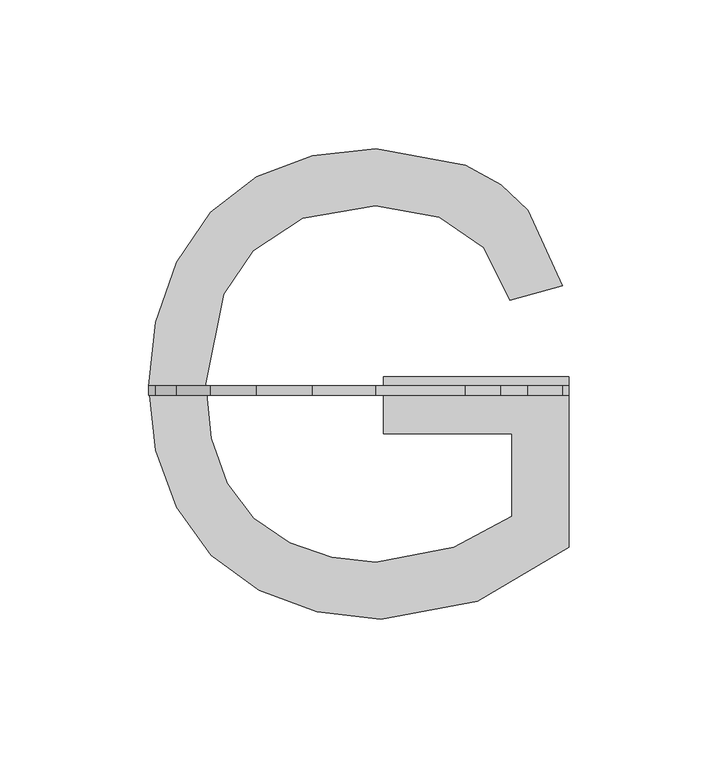
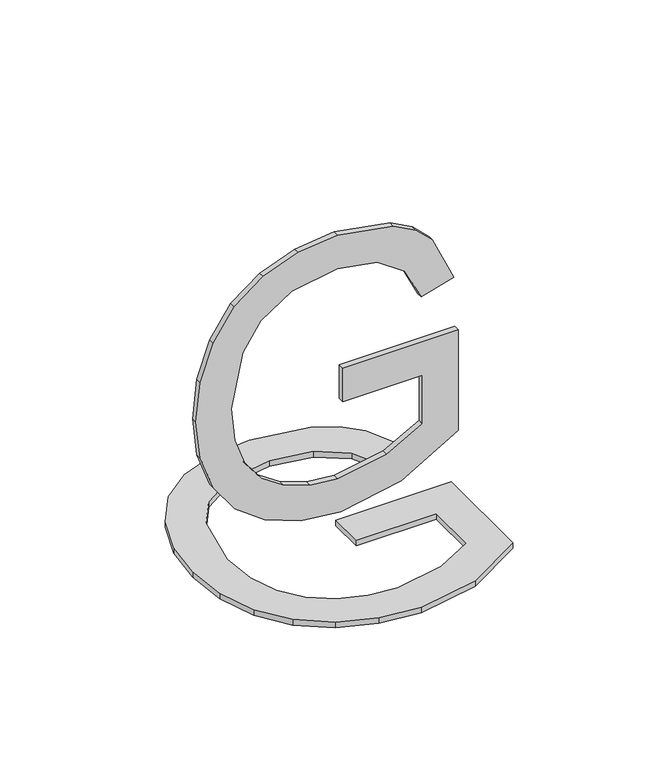
"""IFC4 building model written with IfcOpenShell, lengths in millimetres: proxy geometry, Grid Number1_FedEx : Grid Number1_FedEx."""

from ifc_helpers import new_model, si_unit, frame, origin, origin_with_axes, place, context, project, spatial, polyline, outline, extrude, source, transform, mapped, element, save


def entourage_0d31b632(model_context):
    return source(origin(), model_context, "Body", "SweptSolid", [
        extrude(outline(polyline([(-102.093637, 206.3869621), (-102.093637, 225.5238891), (-39.898624, 225.5238891), (-39.898624, 168.2999919), (-70.603674, 150.2469924), (-103.0654341, 144.191949), (-124.5337398, 146.5980812), (-143.9369766, 153.8164778), (-160.0557262, 165.5948453), (-171.6705702, 181.6808902), (-178.6927385, 200.9766687), (-181.0334612, 222.384237), (-178.7020827, 243.9459847), (-171.707947, 264.0033158), (-160.3407244, 280.8275527), (-144.8900853, 292.690018), (-126.0708611, 299.7262026), (-104.5978833, 302.0715975), (-74.659058, 296.6332715), (-62.721839, 290.1297065), (-53.6719787, 281.4956632), (-42.1038558, 256.1728739), (-59.7457105, 251.2017581), (-68.4731958, 268.899678), (-83.3865433, 279.1035473), (-104.8968978, 282.9346704), (-129.3973972, 278.8045328), (-146.0674548, 267.9652577), (-155.9162444, 253.2201059), (-161.8965342, 223.1691501), (-160.0977751, 204.8685291), (-154.7014981, 189.8103465), (-145.8712266, 178.1020606), (-133.7704841, 169.8511296), (-119.6093449, 164.9594395), (-104.5978833, 163.3288761), (-78.4154274, 168.2439267), (-59.0355511, 178.7281221), (-59.0355511, 206.3869621), (-102.093637, 206.3869621)])), origin_with_axes(), (0.0, 0.0, 1.0), 3.175),
        extrude(outline(polyline([(74.2827904, -102.093637), (74.2827904, -59.0355511), (46.6239505, -59.0355511), (36.1397551, -78.4154274), (31.2247044, -104.5978833), (32.8552678, -119.6093449), (37.7469579, -133.7704841), (45.9978889, -145.8712266), (57.7061748, -154.7014981), (72.7643574, -160.0977751), (91.0649784, -161.8965342), (121.1159342, -155.9162444), (135.861086, -146.0674548), (146.7003611, -129.3973972), (150.8304987, -104.8968978), (146.9993756, -83.3865433), (136.7955063, -68.4731958), (119.0975864, -59.7457105), (124.0687022, -42.1038558), (149.3914915, -53.6719787), (158.0255348, -62.721839), (164.5290998, -74.659058), (169.9674258, -104.5978833), (167.6220309, -126.0708611), (160.5858463, -144.8900853), (148.723381, -160.3407244), (131.8991441, -171.707947), (111.841813, -178.7020827), (90.2800654, -181.0334612), (68.872497, -178.6927385), (49.5767185, -171.6705702), (33.4906736, -160.0557262), (21.7123061, -143.9369766), (14.4939095, -124.5337398), (12.0877774, -103.0654341), (18.1428207, -70.603674), (36.1958203, -39.898624), (93.4197175, -39.898624), (93.4197175, -102.093637), (74.2827904, -102.093637)])), frame((0.0, 219.3456765, 0.0), z_axis=(0.0, 1.0, 0.0), x_axis=(0.0, 0.0, 1.0)), (0.0, 0.0, 1.0), 3.175),
    ])


if __name__ == "__main__":
    model = new_model("IFC4")
    model_context = context("Model", 3, world=origin())
    ifc_project = project(units=[si_unit("LENGTHUNIT", "METRE", prefix="MILLI")], contexts=[model_context])
    site = spatial("IfcSite", under=ifc_project)
    building = spatial("IfcBuilding", under=site)
    placement = place(None, origin())
    entourage_shape = entourage_0d31b632(model_context)
    element("IfcBuildingElementProxy", 1, Name="Grid Number1_FedEx : Grid Number1_FedEx", ObjectType="Grid Number1_FedEx : Grid Number1_FedEx", at=placement, inside=building, context=model_context, shape_type="MappedRepresentation", body=[
        mapped(entourage_shape, transform((0.0, 0.0, 0.0), x_axis=(1.0, 0.0, 0.0), y_axis=(0.0, 1.0, 0.0), z_axis=(0.0, 0.0, 1.0))),
    ])
    save(model, "model.ifc")

# Revit data of these elements
# Type "Grid Number1_FedEx : Grid Number1_FedEx"
#   Grid [instance default] = "S.8"
#   Label Width [instance default] = 1' - 0"
#   Half Box Width2 [instance default] = 0' - 6.13846"
#   Half Box Width [instance default] = 0' - 6"
#   Robust [instance default] = yes
#   Height = 0
#   Assembly Code = ""
# Element 1 (IfcBuildingElementProxy, "Grid Number1_FedEx : Grid Number1_FedEx")
#   Grid = "G"
#   Robust = no
#   Materials on its faces: "Letter"
# Materials
#   "Letter": class "Unassigned", colour RGB 178 187 30, transparency 0, Comments = "Rendering appearance not upgraded "
